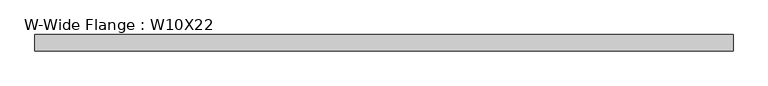
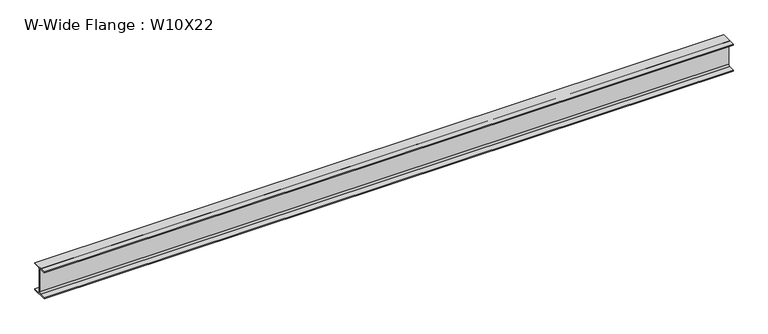
"""IFC4 building model written with IfcOpenShell, lengths in millimetres: beam geometry, W-Wide Flange : W10X22."""

from ifc_helpers import new_model, si_unit, point, frame, frame_2d, origin, place, context, project, spatial, polyline, circle_curve, trimmed, segment, composite_curve, outline, extrude, source, transform, mapped, element, save


def w_wide_flange_w10x22_a828ce3f(model_context):
    return source(origin(), model_context, "Body", "SweptSolid", [
        extrude(outline(composite_curve([segment(polyline([(-73.025, -120.396), (-17.7165, -120.396)]), True, "CONTINUOUS"), segment(trimmed(circle_curve(frame_2d((-17.7165, -105.7275)), 14.6685), [point((-17.7165, -120.396))], [point((-3.048, -105.7275))], True, "CARTESIAN"), True, "CONTINUOUS"), segment(polyline([(-3.048, -105.7275), (-3.048, 105.7275)]), True, "CONTINUOUS"), segment(trimmed(circle_curve(frame_2d((-17.7165, 105.7275)), 14.6685), [point((-3.048, 105.7275))], [point((-17.7165, 120.396))], True, "CARTESIAN"), True, "CONTINUOUS"), segment(polyline([(-17.7165, 120.396), (-73.025, 120.396), (-73.025, 129.54), (73.025, 129.54), (73.025, 120.396), (17.7165, 120.396)]), True, "CONTINUOUS"), segment(trimmed(circle_curve(frame_2d((17.7165, 105.7275)), 14.6685), [point((17.7165, 120.396))], [point((3.048, 105.7275))], True, "CARTESIAN"), True, "CONTINUOUS"), segment(polyline([(3.048, 105.7275), (3.048, -105.7275)]), True, "CONTINUOUS"), segment(trimmed(circle_curve(frame_2d((17.7165, -105.7275)), 14.6685), [point((3.048, -105.7275))], [point((17.7165, -120.396))], True, "CARTESIAN"), True, "CONTINUOUS"), segment(polyline([(17.7165, -120.396), (73.025, -120.396), (73.025, -129.54), (-73.025, -129.54), (-73.025, -120.396)]), True, "CONTINUOUS")], self_intersect=False)), frame((-3121.025, 0.0, 0.0), z_axis=(1.0, 0.0, 0.0), x_axis=(0.0, 1.0, 0.0)), (0.0, 0.0, 1.0), 6242.05),
    ])


if __name__ == "__main__":
    model = new_model("IFC4")
    model_context = context("Model", 3, world=origin())
    ifc_project = project(units=[si_unit("LENGTHUNIT", "METRE", prefix="MILLI")], contexts=[model_context])
    site = spatial("IfcSite", under=ifc_project)
    building = spatial("IfcBuilding", under=site)
    placement = place(None, origin())
    w_wide_flange_w10x22_shape = w_wide_flange_w10x22_a828ce3f(model_context)
    element("IfcBeam", 1, ObjectType="W-Wide Flange : W10X22", at=placement, inside=building, context=model_context, shape_type="MappedRepresentation", body=[
        mapped(w_wide_flange_w10x22_shape, transform((0.0, 0.0, 0.0), x_axis=(1.0, 0.0, 0.0), y_axis=(0.0, 1.0, 0.0), z_axis=(0.0, 0.0, 1.0))),
    ])
    save(model, "model.ifc")

# Revit data of these elements
# Type "W-Wide Flange : W10X22"
#   Assembly Code = "B10"
#   W = 22
#   Length [instance default] = 5' - 0"
#   bf = 0' - 5 3/4"
#   d = 0' - 10.2"
#   k = 0' - 0 15/16"
#   k2 = 0' - 0.5775"
#   tf = 0' - 0.36"
#   tw = 0' - 0.24"
#   A = 0.0450694 SF
#   Structural Material [instance default] = Steel ASTM A992
# Element 1 (IfcBeam, "W-Wide Flange : W10X22")
#   Structural Material = none
# Materials
#   "Steel ASTM A992": class "Metal", colour RGB 189 187 185, transparency 0, Description = "Structural steel 50ksi", Cost = 0
